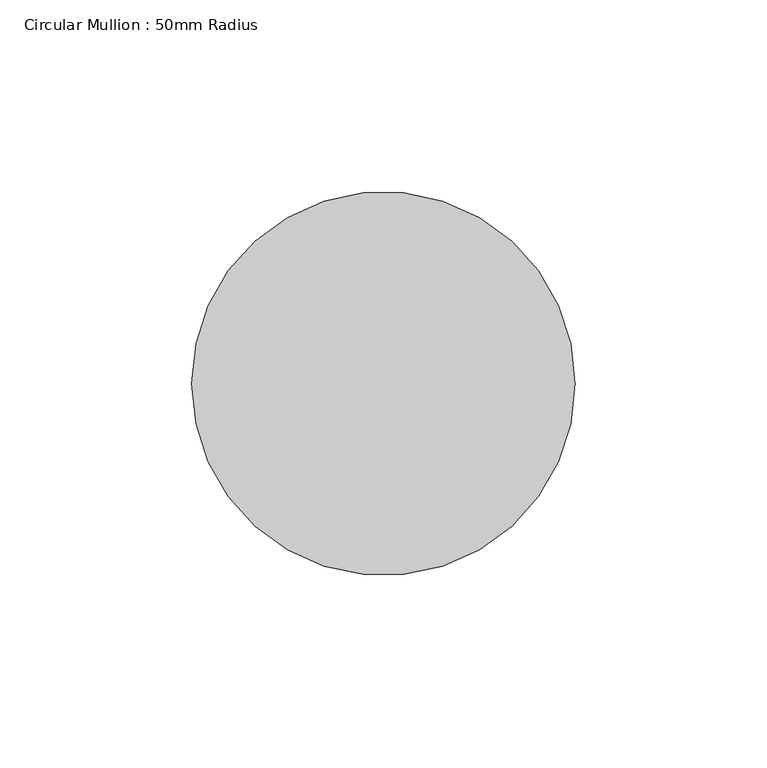
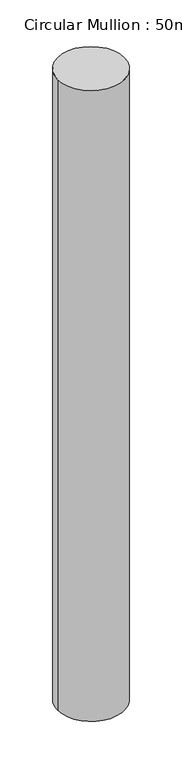
"""IFC4 building model written with IfcOpenShell, lengths in millimetres: member geometry, Circular Mullion : 50mm Radius."""

from ifc_helpers import new_model, si_unit, point, frame, origin, origin_2d, place, context, project, spatial, circle_curve, trimmed, segment, composite_curve, outline, extrude, source, transform, mapped, element, save


def circular_mullion_50mm_radius_1e17e15d(model_context):
    return source(origin(), model_context, "Body", "SweptSolid", [
        extrude(outline(composite_curve([segment(trimmed(circle_curve(origin_2d(), 50.0), [point((50.0, 0.0))], [point((-50.0, 0.0))], False, "CARTESIAN"), True, "CONTINUOUS"), segment(trimmed(circle_curve(origin_2d(), 50.0), [point((-50.0, 0.0))], [point((50.0, 0.0))], False, "CARTESIAN"), True, "CONTINUOUS")], self_intersect=False)), frame((0.0, 0.0, -1001.2127307), z_axis=(0.0, 0.0, 1.0), x_axis=(1.0, 0.0, 0.0)), (0.0, 0.0, 1.0), 1001.2127307),
    ])


if __name__ == "__main__":
    model = new_model("IFC4")
    model_context = context("Model", 3, world=origin())
    ifc_project = project(units=[si_unit("LENGTHUNIT", "METRE", prefix="MILLI")], contexts=[model_context])
    site = spatial("IfcSite", under=ifc_project)
    building = spatial("IfcBuilding", under=site)
    placement = place(None, origin())
    circular_mullion_50mm_radius_shape = circular_mullion_50mm_radius_1e17e15d(model_context)
    element("IfcMember", 1, ObjectType="Circular Mullion : 50mm Radius", at=placement, inside=building, context=model_context, shape_type="MappedRepresentation", body=[
        mapped(circular_mullion_50mm_radius_shape, transform((0.0, 0.0, 0.0), x_axis=(1.0, 0.0, 0.0), y_axis=(0.0, 1.0, 0.0), z_axis=(0.0, 0.0, 1.0))),
    ])
    save(model, "model.ifc")

# Revit data of these elements
# Type "Circular Mullion : 50mm Radius"
#   built-in parameter 1007350 = 0.164042 (stored number, unit not read)
# Element 1 (IfcMember, "Circular Mullion : 50mm Radius")
#   Materials on its faces: "Aluminium"
# Materials
#   "Aluminium": class "Metal", colour RGB 247 247 247, transparency 0, Description = "Aluminium 6061", Cost = 0
